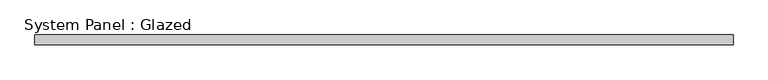
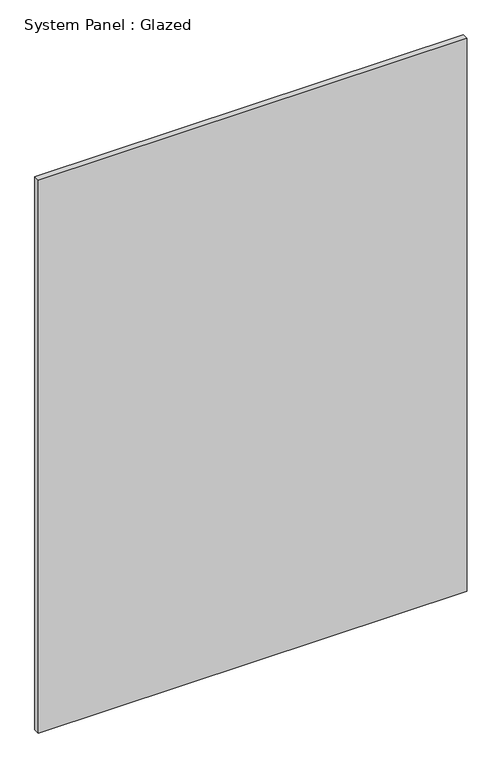
"""IFC4 building model written with IfcOpenShell, lengths in millimetres: plate geometry, System Panel : Glazed."""

from ifc_helpers import new_model, si_unit, origin, origin_with_axes, place, context, project, spatial, polyline, outline, extrude, source, transform, mapped, element, save


def system_panel_glazed_6831b779(model_context):
    return source(origin(), model_context, "Body", "SweptSolid", [
        extrude(outline(polyline([(890.0, -49.5), (-890.0, -49.5), (-890.0, -24.5), (890.0, -24.5), (890.0, -49.5)])), origin_with_axes(), (0.0, 0.0, 1.0), 2425.0),
    ])


if __name__ == "__main__":
    model = new_model("IFC4")
    model_context = context("Model", 3, world=origin())
    ifc_project = project(units=[si_unit("LENGTHUNIT", "METRE", prefix="MILLI")], contexts=[model_context])
    site = spatial("IfcSite", under=ifc_project)
    building = spatial("IfcBuilding", under=site)
    placement = place(None, origin())
    system_panel_glazed_shape = system_panel_glazed_6831b779(model_context)
    element("IfcPlate", 1, ObjectType="System Panel : Glazed", at=placement, inside=building, context=model_context, shape_type="MappedRepresentation", body=[
        mapped(system_panel_glazed_shape, transform((0.0, 0.0, 0.0), x_axis=(1.0, 0.0, 0.0), y_axis=(0.0, 1.0, 0.0), z_axis=(0.0, 0.0, 1.0))),
    ])
    save(model, "model.ifc")

# Revit data of these elements
# Type "System Panel : Glazed"
#   Keynote = "H11"
#   Construction Type Id = "GSP4R"
#   Analytic Construction = "1/8 in Pilkington single glazing"
#   Visual Light Transmittance = 0.9
#   Solar Heat Gain Coefficient = 0.86
#   Heat Transfer Coefficient (U) = 6.7069 W/(m²·K)
# Element 1 (IfcPlate, "System Panel : Glazed")
#   Materials on its faces: "Glass"
# Materials
#   "Glass": class "Glass", colour RGB 0 128 192, transparency 0.9, Description = "Soda Lime Glass", Cost = 0
